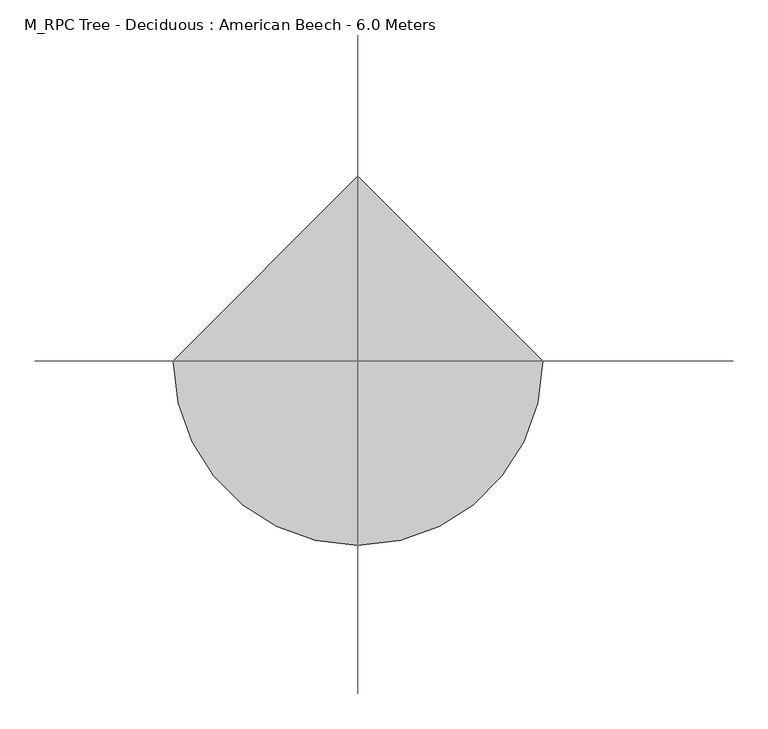
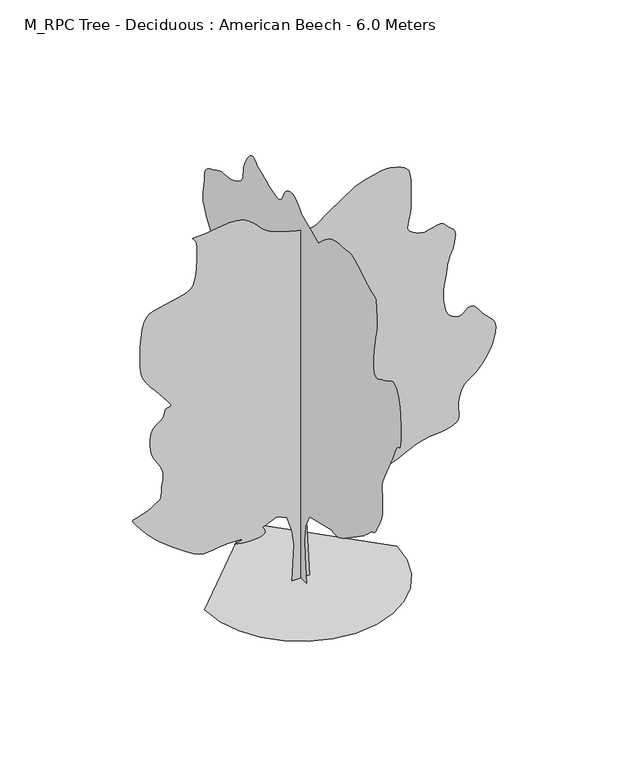
"""IFC4 building model written with IfcOpenShell, lengths in millimetres: geographic element geometry, M_RPC Tree - Deciduous : American Beech - 6.0 Meters."""

from ifc_helpers import new_model, si_unit, origin, place, context, project, spatial, triangles, source, transform, mapped, element, save


def m_rpc_tree_deciduous_american_beech_6_0_meters_be49fed4(model_context):
    return source(origin(), model_context, "Body", "Tessellation", [
        triangles([(0.0009733, 134.7013619, 0.0), (0.0009733, -147.494867, 0.0), (0.0009733, -109.8685844, 413.8878181), (0.0009733, -100.4623272, 649.050499), (0.0009733, -119.2748508, 884.2131798), (0.0009733, -232.153435, 1100.5634188), (0.0009733, -805.9506603, 1241.6609837), (0.0009733, -836.5581671, 1230.0334957), (0.0009733, -869.3831984, 1221.2035114), (0.0009733, -906.6532345, 1217.965991), (0.0009733, -950.5882708, 1223.1234524), (0.0009733, -1003.4058317, 1239.4685303), (0.0009733, -1067.3308542, 1269.7985104), (0.0009733, -1144.5859497, 1316.9135124), (0.0009733, -1455.0011593, 1533.2636787), (0.0009733, -1498.8811844, 1564.1163013), (0.0009733, -1542.2661816, 1593.486311), (0.0009733, -1585.8162849, 1623.3513485), (0.0009733, -1630.1888672, 1655.6862934), (0.0009733, -1676.041301, 1692.4613743), (0.0009733, -1724.0338657, 1735.6539413), (0.0009733, -1774.8239342, 1787.2388741), (0.0009733, -1818.8389801, 1828.7590141), (0.0009733, -1849.3615356, 1847.5739994), (0.0009733, -1871.3289448, 1854.3740204), (0.0009733, -1889.6765167, 1859.8590054), (0.0009733, -1909.3389793, 1874.7240864), (0.0009733, -1935.2541126, 1909.6614887), (0.0009733, -1972.3591152, 1975.3715767), (0.0009733, -2012.7566494, 2050.40159), (0.0009733, -2045.5841515, 2111.4491718), (0.0009733, -2071.3341785, 2166.4067184), (0.0009733, -2090.5042294, 2223.1767998), (0.0009733, -2103.5867157, 2289.651812), (0.0009733, -2111.0717239, 2373.7344704), (0.0009733, -2113.4592236, 2483.3219673), (0.0009733, -2108.7967175, 2583.5521866), (0.0009733, -2099.1991928, 2645.9521568), (0.0009733, -2091.2441551, 2687.927211), (0.0009733, -2091.5191383, 2726.9521545), (0.0009733, -2106.6016479, 2780.4523773), (0.0009733, -2143.0767471, 2865.9023941), (0.0009733, -2207.5242668, 3000.6773071), (0.0009733, -2272.3543213, 3131.8524399), (0.0009733, -2311.5169018, 3208.0527306), (0.0009733, -2333.894315, 3249.2275429), (0.0009733, -2348.3743904, 3275.2526985), (0.0009733, -2363.8419056, 3306.0525627), (0.0009733, -2389.1819286, 3361.5276649), (0.0009733, -2433.2795277, 3461.6026611), (0.0009733, -2483.0818657, 3552.8029083), (0.0009733, -2520.7019531, 3587.7528099), (0.0009733, -2547.8020432, 3595.3779259), (0.0009733, -2566.002095, 3604.6529411), (0.0009733, -2576.9770065, 3644.5278328), (0.0009733, -2582.3519691, 3743.9531593), (0.0009733, -2583.7771729, 3931.9283134), (0.0009733, -2574.1771774, 4144.4034256), (0.0009733, -2548.4520035, 4302.6033623), (0.0009733, -2511.2269501, 4413.2285866), (0.0009733, -2467.0668549, 4483.053685), (0.0009733, -2420.6095161, 4518.8035378), (0.0009733, -2376.4569786, 4527.2536034), (0.0009733, -2339.2143391, 4515.1287621), (0.0009733, -2306.9368034, 4495.0285355), (0.0009733, -2274.4943069, 4475.2535797), (0.0009733, -2241.7217434, 4456.1535828), (0.0009733, -2208.456768, 4438.0035278), (0.0009733, -2174.5318039, 4421.2036812), (0.0009733, -2139.7866863, 4406.0284447), (0.0009733, -2104.0516582, 4392.8536674), (0.0009733, -2063.4092262, 4373.6786751), (0.0009733, -2017.3366024, 4348.9034431), (0.0009733, -1970.769096, 4331.3786407), (0.0009733, -1928.6465218, 4333.9284851), (0.0009733, -1895.9015728, 4369.4036453), (0.0009733, -1877.4714478, 4450.6036308), (0.0009733, -1878.294072, 4590.37882), (0.0009733, -1893.3515831, 4743.5287743), (0.0009733, -1912.3565277, 4862.9290443), (0.0009733, -1932.3490574, 4958.6287262), (0.0009733, -1950.3665623, 5040.6789505), (0.0009733, -1963.4490486, 5119.1293945), (0.0009733, -1968.6315811, 5203.9794479), (0.0009733, -1962.9540207, 5305.2790787), (0.0009733, -1955.0840069, 5402.479541), (0.0009733, -1951.8190899, 5472.3543457), (0.0009733, -1947.4040977, 5521.0042831), (0.0009733, -1936.0790623, 5554.5045639), (0.0009733, -1912.0815445, 5578.9792328), (0.0009733, -1869.6565178, 5600.4796646), (0.0009733, -1803.044014, 5625.1043243), (0.0009733, -1720.9064404, 5661.3794357), (0.0009733, -1636.6338226, 5709.179425), (0.0009733, -1551.5337845, 5761.6047134), (0.0009733, -1466.931245, 5811.7045624), (0.0009733, -1384.1386242, 5852.5799744), (0.0009733, -1304.4711033, 5877.3546249), (0.0009733, -1229.2460438, 5879.0795197), (0.0009733, -1155.7484224, 5869.4295273), (0.0009733, -1081.2633614, 5862.9049255), (0.0009733, -1007.1082947, 5856.8547134), (0.0009733, -934.5982584, 5848.679631), (0.0009733, -865.0506866, 5835.7548386), (0.0009733, -799.7806154, 5815.4049179), (0.0009733, -740.1056242, 5785.0044479), (0.0009733, -686.9580688, 5749.2798843), (0.0009733, -639.7330444, 5714.5296799), (0.0009733, -597.445473, 5680.604425), (0.0009733, -559.105444, 5647.3547104), (0.0009733, -523.727916, 5614.5793854), (0.0009733, -490.3254127, 5582.1296219), (0.0009733, -457.9103854, 5549.8542664), (0.0009733, -15.8033629, 5737.9794113), (0.0009733, 22.480868, 5779.9547562), (0.0009733, 60.6828013, 5819.9046432), (0.0009733, 98.7203278, 5855.7047836), (0.0009733, 136.5108627, 5885.354718), (0.0009733, 173.9723933, 5906.7795731), (0.0009733, 211.0226754, 5917.9050568), (0.0009733, 247.5792013, 5916.7045486), (0.0009733, 282.6827272, 5907.9045044), (0.0009733, 315.3177446, 5896.9545914), (0.0009733, 345.3202738, 5882.8798691), (0.0009733, 372.5252993, 5864.7048157), (0.0009733, 396.7678239, 5841.4294922), (0.0009733, 417.8828505, 5812.054541), (0.0009733, 435.7103597, 5775.6044403), (0.0009733, 452.7128829, 5735.1795822), (0.0009733, 472.6778707, 5696.4046234), (0.0009733, 497.4153869, 5662.079393), (0.0009733, 528.7329157, 5634.979303), (0.0009733, 568.4429555, 5617.9047638), (0.0009733, 618.3554976, 5613.7044388), (0.0009733, 680.2805695, 5625.1043243), (0.0009733, 747.7156248, 5646.6297546), (0.0009733, 813.1781261, 5670.6294525), (0.0009733, 876.993199, 5696.6796066), (0.0009733, 939.4932358, 5724.37966), (0.0009733, 1001.0058329, 5753.3046387), (0.0009733, 1061.8608393, 5783.054567), (0.0009733, 1122.385924, 5813.2294693), (0.0009733, 1150.6609423, 5838.9296448), (0.0009733, 1179.2634842, 5861.5800064), (0.0009733, 1208.5259422, 5878.1545761), (0.0009733, 1238.7735146, 5885.5797043), (0.0009733, 1270.3410645, 5880.8299942), (0.0009733, 1303.5511013, 5860.8794678), (0.0009733, 1338.7360176, 5822.6294769), (0.0009733, 1373.2086227, 5775.8044281), (0.0009733, 1403.7311783, 5731.2548218), (0.0009733, 1429.8111271, 5687.8795624), (0.0009733, 1450.9562027, 5644.4793045), (0.0009733, 1466.6712318, 5599.9546967), (0.0009733, 1476.4611866, 5553.1046494), (0.0009733, 1479.8336552, 5502.8042313), (0.0009733, 1483.4812523, 5452.1044189), (0.0009733, 1495.191148, 5404.7044052), (0.0009733, 1516.1161789, 5360.4042023), (0.0009733, 1547.4087456, 5319.0793991), (0.0009733, 1590.2163071, 5280.554425), (0.0009733, 1645.6963509, 5244.6542908), (0.0009733, 1714.996336, 5211.204007), (0.0009733, 1788.9065048, 5186.2043701), (0.0009733, 1858.2064899, 5172.3790512), (0.0009733, 1924.0515987, 5164.8039322), (0.0009733, 1987.5940865, 5158.5543137), (0.0009733, 2049.9841736, 5148.679335), (0.0009733, 2112.3742607, 5130.2542969), (0.0009733, 2175.9167484, 5098.32892), (0.0009733, 2240.5017597, 5064.3292511), (0.0009733, 2303.2743816, 5038.2291), (0.0009733, 2361.2769459, 5012.9289001), (0.0009733, 2411.5469879, 4981.4040802), (0.0009733, 2451.1195724, 4936.5289124), (0.0009733, 2477.0345604, 4871.2538269), (0.0009733, 2486.331958, 4778.503965), (0.0009733, 2492.5844833, 4683.078685), (0.0009733, 2506.4019539, 4608.2036041), (0.0009733, 2520.4019714, 4544.5287117), (0.0009733, 2527.1521408, 4482.6537094), (0.0009733, 2519.2520416, 4413.2285866), (0.0009733, 2489.2945679, 4326.8286278), (0.0009733, 2429.8919437, 4214.1285301), (0.0009733, 2356.3968658, 4101.0031677), (0.0009733, 2289.9743214, 4014.028244), (0.0009733, 2231.9442879, 3944.8531059), (0.0009733, 2183.6218014, 3885.0282692), (0.0009733, 2146.3266941, 3826.2030807), (0.0009733, 2121.3692059, 3759.9780533), (0.0009733, 2110.0716396, 3677.9528275), (0.0009733, 2115.5842392, 3588.602758), (0.0009733, 2136.8916595, 3505.6778778), (0.0009733, 2169.0617889, 3428.6526375), (0.0009733, 2207.1542313, 3357.0776459), (0.0009733, 2246.2317879, 3290.4526428), (0.0009733, 2281.3643818, 3228.2526604), (0.0009733, 2307.6092915, 3170.0024368), (0.0009733, 2333.0293968, 3130.6025162), (0.0009733, 2364.704353, 3115.0525932), (0.0009733, 2396.2144936, 3108.0524391), (0.0009733, 2421.1445126, 3094.3024063), (0.0009733, 2433.074453, 3058.5275551), (0.0009733, 2425.586974, 2985.3773689), (0.0009733, 2392.2669147, 2859.5771988), (0.0009733, 2346.3593971, 2717.8521286), (0.0009733, 2303.741795, 2602.2772064), (0.0009733, 2261.946817, 2505.6519997), (0.0009733, 2218.506736, 2420.6845116), (0.0009733, 2170.9542606, 2340.1668972), (0.0009733, 2116.8167221, 2256.8517792), (0.0009733, 2053.6316254, 2163.5018085), (0.0009733, 1990.2540985, 2069.4091507), (0.0009733, 1937.0790012, 1987.8215435), (0.0009733, 1893.941518, 1917.4240963), (0.0009733, 1860.6740719, 1856.8965408), (0.0009733, 1837.1164982, 1804.928928), (0.0009733, 1823.1039814, 1760.1989548), (0.0009733, 1818.4689445, 1721.3939106), (0.0009733, 1822.4189941, 1694.76385), (0.0009733, 1831.633984, 1682.286414), (0.0009733, 1842.1640099, 1676.2263187), (0.0009733, 1850.0614929, 1668.8488621), (0.0009733, 1851.3789997, 1652.4213764), (0.0009733, 1842.1640099, 1619.2113396), (0.0009733, 1818.4689445, 1561.4837585), (0.0009733, 1798.7513981, 1500.5736683), (0.0009733, 1796.6388817, 1458.9161819), (0.0009733, 1800.9439968, 1430.4235897), (0.0009733, 1800.4789089, 1409.0036762), (0.0009733, 1784.0514233, 1388.5736732), (0.0009733, 1740.4738506, 1363.0410748), (0.0009733, 1658.5587925, 1326.3210777), (0.0009733, 1569.2912762, 1288.8036003), (0.0009733, 1504.2137077, 1262.3110313), (0.0009733, 1452.9586967, 1242.8959373), (0.0009733, 1405.1587074, 1226.6059433), (0.0009733, 1350.4460587, 1209.4934704), (0.0009733, 1278.4585922, 1187.608469), (0.0009733, 1178.8259382, 1157.003433), (0.0009733, 1078.8083513, 1127.6584219), (0.0009733, 1006.4358067, 1109.9959099), (0.0009733, 952.4932417, 1100.7283796), (0.0009733, 907.7632685, 1096.558358), (0.0009733, 863.0356934, 1094.2008711), (0.0009733, 809.0906576, 1090.3609165), (0.0009733, 736.7181129, 1081.7509043), (0.0009733, 652.0605623, 1068.0108273), (0.0009733, 567.4004683, 1051.3083584), (0.0009733, 482.7428813, 1032.140851), (0.0009733, 398.0828236, 1010.9958481), (0.0009733, 313.4252366, 988.3707756), (0.0009733, 228.7664324, 964.7582634), (0.0009733, 144.1076192, 940.6532667), (134.0396109, 0.0003104, 0.0138465), (-129.3426047, 0.0003104, 0.0138465), (-101.123079, 0.0002775, 554.9979549), (-129.3426047, 0.000265, 780.7556139), (-204.5949064, 0.0002508, 1015.9182947), (-355.1002728, 0.0002461, 1091.1708961), (-571.4504754, 0.0002508, 997.1057802), (-553.8429382, 0.0002524, 972.9983128), (-539.4454522, 0.000254, 949.3882713), (-531.465416, 0.0002555, 926.7632715), (-533.1104465, 0.0002571, 905.6181959), (-547.5904492, 0.0002587, 886.4482178), (-578.1129684, 0.0002587, 869.7482197), (-627.8879826, 0.0002602, 856.0082153), (-686.4380424, 0.0002602, 846.9307171), (-741.5356241, 0.0002602, 843.2831926), (-793.7506056, 0.0002602, 844.1606827), (-843.663184, 0.0002602, 848.6581553), (-891.8482515, 0.0002602, 855.8707237), (-938.8807732, 0.0002587, 864.8932108), (-985.3357864, 0.0002587, 874.8207298), (-938.2757229, 0.0002587, 886.8056814), (-899.1157585, 0.0002571, 898.1307169), (-875.7482168, 0.0002571, 908.1407164), (-876.0782112, 0.0002555, 916.1757637), (-908.000754, 0.0002555, 921.5782682), (-979.4132555, 0.0002555, 923.690712), (-1098.2134169, 0.0002555, 921.8532515), (-1223.378524, 0.0002571, 913.21577), (-1316.2934921, 0.0002571, 899.9682501), (-1388.4736794, 0.0002571, 889.0257494), (-1451.4387314, 0.0002571, 887.2982386), (-1516.7087299, 0.0002571, 901.6957609), (-1595.8012859, 0.0002555, 939.1307579), (-1700.2313942, 0.0002508, 1006.5108021), (-1816.016478, 0.0002461, 1088.4284037), (-1921.6016029, 0.0002414, 1165.4084433), (-2017.1466431, 0.0002367, 1238.2735451), (-2102.8191753, 0.0002336, 1307.8509842), (-2178.7867767, 0.0002289, 1374.9560452), (-2245.2068504, 0.0002242, 1440.4186192), (-2302.2492989, 0.0002211, 1505.0587143), (-2354.1368294, 0.0002179, 1567.5838223), (-2402.8969345, 0.0002132, 1625.1763824), (-2445.4045143, 0.0002101, 1676.3488403), (-2478.5321434, 0.0002085, 1719.6239605), (-2499.1544312, 0.0002069, 1753.5214554), (-2504.1520912, 0.0002054, 1776.5590027), (-2490.3793854, 0.0002038, 1787.2539894), (-2459.3920326, 0.0002038, 1794.0263958), (-2417.5419708, 0.0002038, 1805.7364368), (-2368.9443558, 0.0002022, 1821.5614883), (-2317.716814, 0.0002007, 1840.6764553), (-2267.9692692, 0.0001991, 1862.2590042), (-2223.8167316, 0.0001991, 1885.4865108), (-2189.3717411, 0.0001975, 1909.5391125), (-2162.3867603, 0.000196, 1927.8015152), (-2138.1966671, 0.000196, 1938.169051), (-2117.2992508, 0.0001944, 1946.561562), (-2100.1866325, 0.0001944, 1958.9016518), (-2087.3541309, 0.0001928, 1981.1165749), (-2079.291687, 0.0001897, 2019.1266094), (-2076.4941833, 0.0001866, 2078.8566845), (-2072.5992176, 0.0001834, 2146.7042873), (-2063.7692333, 0.0001787, 2206.9817127), (-2054.2791149, 0.0001756, 2262.4893711), (-2048.4115952, 0.0001725, 2316.0218594), (-2050.4417038, 0.0001693, 2370.3769718), (-2064.6466507, 0.0001662, 2428.3494507), (-2095.3066978, 0.0001615, 2492.7420319), (-2134.2492336, 0.0001583, 2555.8271347), (-2169.5717869, 0.0001552, 2611.5022247), (-2199.9567055, 0.0001521, 2665.0271553), (-2224.0918602, 0.0001489, 2721.6771858), (-2240.6543667, 0.0001442, 2786.727285), (-2248.3342758, 0.0001395, 2865.4274231), (-2245.8117554, 0.0001348, 2963.0772766), (-2228.8892418, 0.0001286, 3053.9275452), (-2197.981826, 0.0001254, 3115.1525871), (-2158.6842247, 0.0001223, 3156.3276901), (-2116.5866489, 0.0001207, 3186.952565), (-2077.289193, 0.0001191, 3216.6024994), (-2046.3816319, 0.000116, 3254.8024933), (-2029.4615891, 0.0001129, 3311.1025452), (-2011.7716805, 0.0001113, 3359.2778023), (-1982.4016708, 0.0001097, 3377.3028648), (-1952.6991234, 0.0001097, 3381.2026268), (-1934.0241005, 0.0001082, 3386.9028603), (-1937.7266361, 0.0001082, 3410.3778809), (-1975.1615604, 0.0001035, 3467.6028763), (-2057.6791981, 9.72e-05, 3574.5027466), (-2156.9017754, 9.09e-05, 3694.6029739), (-2237.5292667, 8.47e-05, 3789.0530228), (-2300.5494026, 8e-05, 3870.1780128), (-2346.9519482, 7.53e-05, 3950.303064), (-2377.7218723, 7.05e-05, 4041.8032928), (-2393.8469055, 6.27e-05, 4156.9782394), (-2396.3144875, 5.33e-05, 4308.2036018), (-2391.2694466, 4.39e-05, 4470.0786049), (-2382.4394623, 3.61e-05, 4609.2538307), (-2367.1893757, 2.98e-05, 4726.0536781), (-2342.8918762, 2.35e-05, 4820.8039993), (-2306.911805, 1.88e-05, 4893.8541916), (-2256.6142937, 1.57e-05, 4945.4789474), (-2189.3717411, 1.41e-05, 4976.0538254), (-2104.7392616, 1.25e-05, 4994.8788391), (-2008.7541321, 1.25e-05, 5012.5289246), (-1908.491502, 1.1e-05, 5031.3539383), (-1811.0265209, 9.4e-06, 5053.6293228), (-1723.4339024, 7.8e-06, 5081.6543564), (-1652.7887959, 6.3e-06, 5117.7288986), (-1606.1663509, 3.1e-06, 5164.2039688), (-1578.8513031, -1.6e-06, 5232.7044388), (-1560.4237942, -6.3e-06, 5326.3795349), (-1549.3987404, -1.25e-05, 5434.7043182), (-1544.298761, -2.04e-05, 5547.1544312), (-1543.6387722, -2.67e-05, 5653.1793549), (-1545.9437187, -3.14e-05, 5742.2547318), (-1549.7288074, -3.45e-05, 5803.8294617), (-1560.9438206, -3.76e-05, 5842.6799973), (-1580.7187763, -3.92e-05, 5871.4799835), (-1600.3263004, -4.08e-05, 5891.7049118), (-1611.0487564, -4.08e-05, 5904.879689), (-1604.1663277, -4.23e-05, 5912.4298096), (-1570.95382, -4.23e-05, 5915.9045975), (-1502.6962132, -4.23e-05, 5916.7295471), (-1406.2711395, -4.23e-05, 5923.0547424), (-1298.001004, -4.39e-05, 5937.4550262), (-1183.3109842, -4.39e-05, 5953.0046585), (-1067.6358501, -4.39e-05, 5962.7796432), (-956.4032501, -4.39e-05, 5959.9048187), (-855.043158, -4.39e-05, 5937.4550262), (-768.9856201, -4.08e-05, 5888.5045258), (-703.6355392, -3.61e-05, 5829.3546478), (-655.0655388, -3.29e-05, 5779.2298004), (-614.7254866, -3.14e-05, 5735.7045502), (-574.0554763, -2.82e-05, 5696.3046295), (-524.5004342, -2.67e-05, 5658.5546082), (-457.5028522, -2.35e-05, 5619.9546387), (-364.5052946, -2.19e-05, 5578.0792877), (-256.7552037, -1.88e-05, 5538.7543625), (-153.2841212, -1.72e-05, 5508.8044464), (-57.2167973, -1.57e-05, 5487.254599), (28.3195219, -1.57e-05, 5473.1042999), (100.1988349, -1.57e-05, 5465.3791901), (155.2941184, -1.41e-05, 5463.054332), (190.4793981, -1.57e-05, 5465.2042007), (215.8194211, -1.57e-05, 5473.054303), (243.4629554, -1.57e-05, 5487.6295761), (273.410219, -1.72e-05, 5507.6545166), (305.6602309, -1.88e-05, 5531.7792068), (340.2152802, -2.04e-05, 5558.729306), (377.0728051, -2.19e-05, 5587.1293167), (416.2353493, -2.35e-05, 5615.7043167), (792.4981384, -3.92e-05, 5869.679512), (817.288195, -3.92e-05, 5878.9295288), (882.5581936, -4.08e-05, 5902.1548553), (974.6482847, -4.23e-05, 5932.6297394), (1079.9033426, -4.55e-05, 5963.5795944), (1184.6634453, -4.55e-05, 5988.3048294), (1275.2734669, -4.7e-05, 6000.0046967), (1338.0760288, -4.7e-05, 5991.9796051), (1385.3260517, -4.55e-05, 5975.0550568), (1436.1986732, -4.39e-05, 5961.4297256), (1487.4012165, -4.39e-05, 5946.3050674), (1535.6386791, -4.23e-05, 5924.9546265), (1577.6262325, -4.08e-05, 5892.5548599), (1610.068729, -3.76e-05, 5844.3798935), (1629.6788692, -3.29e-05, 5775.6294388), (1639.0838184, -2.82e-05, 5698.6044891), (1643.8838161, -2.51e-05, 5627.2047775), (1645.2263214, -2.04e-05, 5558.9042953), (1644.2663509, -1.72e-05, 5491.2793533), (1642.1538345, -1.25e-05, 5421.8545212), (1640.0437889, -7.8e-06, 5348.1293701), (1639.0838184, -3.1e-06, 5267.6790482), (1634.0913906, 1.6e-06, 5187.5792862), (1622.1912449, 6.3e-06, 5116.5539703), (1607.9838272, 9.4e-06, 5054.4042755), (1596.081356, 1.25e-05, 5001.0040466), (1591.0912537, 1.57e-05, 4956.1288788), (1597.6187622, 1.72e-05, 4919.6537796), (1620.2713039, 1.88e-05, 4891.4037598), (1651.9738747, 2.04e-05, 4868.9289688), (1682.6888603, 2.19e-05, 4849.728978), (1712.5813671, 2.19e-05, 4833.6537964), (1741.8138851, 2.35e-05, 4820.5540146), (1770.5564621, 2.35e-05, 4810.2287727), (1798.9665012, 2.51e-05, 4802.5539505), (1827.213905, 2.51e-05, 4797.3289787), (1863.2490601, 2.51e-05, 4800.3037971), (1911.6264851, 2.35e-05, 4812.9788956), (1967.4066559, 2.35e-05, 4828.9287941), (2025.6565887, 2.19e-05, 4841.7788818), (2081.4366142, 2.19e-05, 4845.0539726), (2129.8141846, 2.35e-05, 4832.3788742), (2165.8491943, 2.51e-05, 4797.3289787), (2195.3593117, 2.67e-05, 4758.0787582), (2225.6892918, 2.82e-05, 4731.9538994), (2254.2093533, 2.98e-05, 4711.4536972), (2278.2892788, 3.14e-05, 4688.9539078), (2295.2918747, 3.29e-05, 4656.9288277), (2302.5869236, 3.61e-05, 4607.7786301), (2297.5418827, 4.08e-05, 4533.9537758), (2283.3617889, 4.55e-05, 4455.6536133), (2265.8943958, 4.86e-05, 4393.6536186), (2246.4493618, 5.17e-05, 4341.2036224), (2226.3468098, 5.49e-05, 4291.5284569), (2206.9042465, 5.8e-05, 4237.9035324), (2189.4342373, 6.27e-05, 4173.6033875), (2175.2567596, 6.74e-05, 4091.8534355), (2162.3117649, 7.21e-05, 4004.3782516), (2148.874213, 7.68e-05, 3925.278138), (2136.7516972, 8.15e-05, 3851.452993), (2127.756752, 8.62e-05, 3779.753009), (2123.6991508, 8.94e-05, 3707.0780846), (2126.3867775, 9.41e-05, 3630.302829), (2137.6292599, 9.88e-05, 3546.2777252), (2155.4842747, 0.0001035, 3469.5027603), (2176.791695, 0.0001066, 3413.652681), (2201.5542824, 0.0001097, 3374.2527603), (2229.7743622, 0.0001113, 3346.8526886), (2261.4493183, 0.0001129, 3327.0277359), (2296.5819122, 0.0001129, 3310.302594), (2335.1669117, 0.0001144, 3292.3025299), (2374.57439, 0.0001144, 3289.8526794), (2413.1620056, 0.0001129, 3313.0777153), (2452.4043777, 0.0001113, 3347.3276596), (2493.7896423, 0.0001097, 3377.9778236), (2538.8020111, 0.0001082, 3390.3276512), (2588.9021507, 0.0001097, 3369.8027412), (2645.5771797, 0.0001144, 3301.7025375), (2706.5522369, 0.0001191, 3218.4776756), (2765.8771042, 0.0001223, 3156.4526825), (2819.5773148, 0.0001254, 3106.9525063), (2863.7772331, 0.0001286, 3061.2523888), (2894.4523956, 0.0001317, 3010.6025734), (2907.702459, 0.0001348, 2946.27743), (2899.552375, 0.0001411, 2859.6021973), (2878.1022308, 0.0001458, 2766.3523659), (2853.5522758, 0.0001505, 2686.1020317), (2825.0272728, 0.0001552, 2615.752256), (2791.7272705, 0.0001583, 2552.1270699), (2752.8273193, 0.0001615, 2492.1121284), (2707.5271774, 0.0001662, 2432.6019527), (2654.9771873, 0.0001693, 2370.4569088), (2600.8270042, 0.0001725, 2317.1443199), (2551.1021324, 0.0001756, 2280.2868313), (2505.6519997, 0.0001772, 2250.9967587), (2464.3344635, 0.0001787, 2220.3917953), (2426.9544777, 0.0001803, 2179.5842571), (2393.3594353, 0.000185, 2119.691692), (2363.3868462, 0.0001897, 2031.8240902), (2347.2343437, 0.000196, 1934.7965824), (2348.1944595, 0.0002007, 1852.2490047), (2355.7344063, 0.0002038, 1782.5363995), (2359.3269196, 0.0002085, 1724.0139542), (2348.4393574, 0.0002116, 1675.0338043), (2312.5418392, 0.0002132, 1633.9512829), (2241.1018684, 0.0002148, 1599.1237576), (2155.26423, 0.0002164, 1575.9487186), (2078.4766205, 0.0002179, 1565.7737583), (2003.661565, 0.0002179, 1560.866209), (1923.7465302, 0.0002179, 1553.4887524), (1831.6565117, 0.0002195, 1535.9111916), (1720.3138893, 0.0002211, 1500.3962082), (1582.6438042, 0.0002258, 1439.2111347), (1432.7436516, 0.0002289, 1368.8411568), (1291.0710491, 0.000232, 1310.483527), (1160.0909626, 0.0002352, 1263.4785473), (1042.2783136, 0.0002383, 1227.1685543), (940.0957426, 0.0002399, 1200.8959574), (856.0131569, 0.0002399, 1184.0009857), (792.4981384, 0.0002414, 1175.8284468), (397.4228348, 0.0002414, 1166.4234249), (105.8200852, 0.0002446, 1119.3909033), (87.0075707, 0.0002587, 865.4131645), (-1430.8636791, 0.0, 0.0118397), (-1393.0361916, -327.8602567, 0.0118397), (-1285.305994, -628.9454762, 0.0118397), (-1116.2958887, -894.633256, 0.0118397), (-894.633256, -1116.2958887, 0.0118397), (-628.9454762, -1285.305994, 0.0118397), (-327.8602567, -1393.0361916, 0.0118397), (6.25e-05, -1430.8636791, 0.0118397), (327.8602567, -1393.0361916, 0.0118397), (628.9454762, -1285.305994, 0.0118397), (894.633256, -1116.2958887, 0.0118397), (1116.2958887, -894.633256, 0.0118397), (1285.305994, -628.9454762, 0.0118397), (1393.0361916, -327.8602567, 0.0118397), (1430.8636791, 0.0001254, 0.0118397), (-0.0001876, 1430.8636791, 0.0118397)], [[1, 2, 3], [254, 1, 3], [254, 3, 4], [254, 4, 5], [254, 5, 6], [53, 54, 55], [52, 53, 55], [201, 202, 203], [201, 203, 204], [200, 201, 204], [222, 223, 224], [52, 55, 56], [200, 204, 205], [199, 200, 205], [253, 254, 6], [221, 222, 224], [221, 224, 225], [229, 230, 231], [229, 231, 232], [228, 229, 232], [228, 232, 233], [227, 228, 233], [252, 253, 6], [221, 225, 226], [220, 221, 226], [199, 205, 206], [198, 199, 206], [62, 63, 64], [61, 62, 64], [61, 64, 65], [60, 61, 65], [60, 65, 66], [59, 60, 66], [59, 66, 67], [59, 67, 68], [58, 59, 68], [58, 68, 69], [58, 69, 70], [57, 58, 70], [57, 70, 71], [57, 71, 72], [57, 72, 73], [57, 73, 74], [56, 57, 74], [52, 56, 74], [51, 52, 74], [50, 51, 74], [50, 74, 75], [49, 50, 75], [48, 49, 75], [47, 48, 75], [46, 47, 75], [45, 46, 75], [44, 45, 75], [43, 44, 75], [42, 43, 75], [42, 75, 76], [41, 42, 76], [227, 233, 234], [226, 227, 234], [220, 226, 234], [219, 220, 234], [219, 234, 235], [219, 235, 236], [219, 236, 237], [218, 219, 237], [218, 237, 238], [218, 238, 239], [218, 239, 240], [217, 218, 240], [217, 240, 241], [217, 241, 242], [217, 242, 243], [217, 243, 244], [217, 244, 245], [217, 245, 246], [216, 217, 246], [216, 246, 247], [215, 216, 247], [215, 247, 248], [251, 252, 6], [88, 89, 90], [88, 90, 91], [87, 88, 91], [87, 91, 92], [86, 87, 92], [86, 92, 93], [85, 86, 93], [84, 85, 93], [84, 93, 94], [83, 84, 94], [82, 83, 94], [81, 82, 94], [81, 94, 95], [80, 81, 95], [80, 95, 96], [80, 96, 97], [80, 97, 98], [80, 98, 99], [80, 99, 100], [80, 100, 101], [80, 101, 102], [80, 102, 103], [80, 103, 104], [80, 104, 105], [80, 105, 106], [80, 106, 107], [80, 107, 108], [80, 108, 109], [80, 109, 110], [80, 110, 111], [80, 111, 112], [79, 80, 112], [79, 112, 113], [78, 79, 113], [77, 78, 113], [76, 77, 113], [41, 76, 113], [40, 41, 113], [40, 113, 114], [39, 40, 114], [198, 206, 207], [197, 198, 207], [196, 197, 207], [196, 207, 208], [195, 196, 208], [195, 208, 209], [195, 209, 210], [195, 210, 211], [194, 195, 211], [194, 211, 212], [194, 212, 213], [193, 194, 213], [193, 213, 214], [214, 215, 248], [193, 214, 248], [193, 248, 249], [192, 193, 249], [192, 249, 250], [192, 250, 251], [192, 251, 6], [192, 6, 7], [191, 192, 7], [190, 191, 7], [189, 190, 7], [38, 39, 114], [37, 38, 114], [36, 37, 114], [35, 36, 114], [34, 35, 114], [33, 34, 114], [32, 33, 114], [31, 32, 114], [30, 31, 114], [29, 30, 114], [28, 29, 114], [27, 28, 114], [26, 27, 114], [25, 26, 114], [24, 25, 114], [23, 24, 114], [22, 23, 114], [21, 22, 114], [20, 21, 114], [19, 20, 114], [18, 19, 114], [17, 18, 114], [16, 17, 114], [15, 16, 114], [14, 15, 114], [13, 14, 114], [12, 13, 114], [11, 12, 114], [10, 11, 114], [9, 10, 114], [8, 9, 114], [7, 8, 114], [189, 7, 114], [188, 189, 114], [188, 114, 115], [188, 115, 116], [188, 116, 117], [188, 117, 118], [188, 118, 119], [188, 119, 120], [188, 120, 121], [146, 147, 148], [145, 146, 148], [144, 145, 148], [144, 148, 149], [143, 144, 149], [143, 149, 150], [142, 143, 150], [142, 150, 151], [142, 151, 152], [141, 142, 152], [141, 152, 153], [141, 153, 154], [141, 154, 155], [141, 155, 156], [140, 141, 156], [140, 156, 157], [139, 140, 157], [138, 139, 157], [138, 157, 158], [137, 138, 158], [137, 158, 159], [136, 137, 159], [135, 136, 159], [135, 159, 160], [134, 135, 160], [134, 160, 161], [174, 175, 176], [173, 174, 176], [173, 176, 177], [172, 173, 177], [171, 172, 177], [171, 177, 178], [170, 171, 178], [170, 178, 179], [169, 170, 179], [168, 169, 179], [167, 168, 179], [166, 167, 179], [165, 166, 179], [165, 179, 180], [165, 180, 181], [165, 181, 182], [165, 182, 183], [165, 183, 184], [165, 184, 185], [165, 185, 186], [165, 186, 187], [164, 165, 187], [164, 187, 188], [163, 164, 188], [162, 163, 188], [161, 162, 188], [134, 161, 188], [133, 134, 188], [132, 133, 188], [125, 126, 127], [124, 125, 127], [124, 127, 128], [123, 124, 128], [122, 123, 128], [121, 122, 128], [121, 128, 129], [121, 129, 130], [121, 130, 131], [188, 121, 131], [132, 188, 131], [274, 275, 276], [531, 255, 256], [531, 256, 257], [531, 257, 258], [531, 258, 259], [530, 531, 259], [376, 377, 378], [376, 378, 379], [375, 376, 379], [273, 274, 276], [273, 276, 277], [375, 379, 380], [374, 375, 380], [273, 277, 278], [272, 273, 278], [301, 302, 303], [301, 303, 304], [300, 301, 304], [300, 304, 305], [299, 300, 305], [299, 305, 306], [298, 299, 306], [298, 306, 307], [297, 298, 307], [297, 307, 308], [271, 272, 278], [296, 297, 308], [296, 308, 309], [373, 374, 380], [373, 380, 381], [372, 373, 381], [295, 296, 309], [295, 309, 310], [294, 295, 310], [294, 310, 311], [294, 311, 312], [294, 312, 313], [293, 294, 313], [293, 313, 314], [292, 293, 314], [271, 278, 279], [291, 292, 314], [530, 259, 260], [372, 381, 382], [371, 372, 382], [291, 314, 315], [290, 291, 315], [371, 382, 383], [370, 371, 383], [370, 383, 384], [369, 370, 384], [369, 384, 385], [369, 385, 386], [369, 386, 387], [369, 387, 388], [369, 388, 389], [369, 389, 390], [368, 369, 390], [368, 390, 391], [367, 368, 391], [367, 391, 392], [367, 392, 393], [366, 367, 393], [366, 393, 394], [270, 271, 279], [366, 394, 395], [338, 339, 340], [338, 340, 341], [289, 290, 315], [483, 484, 485], [483, 485, 486], [482, 483, 486], [481, 482, 486], [481, 486, 487], [480, 481, 487], [288, 289, 315], [287, 288, 315], [286, 287, 315], [285, 286, 315], [284, 285, 315], [283, 284, 315], [282, 283, 315], [282, 315, 316], [281, 282, 316], [281, 316, 317], [281, 317, 318], [281, 318, 319], [281, 319, 320], [280, 281, 320], [280, 320, 321], [279, 280, 321], [279, 321, 322], [480, 487, 488], [264, 265, 266], [263, 264, 266], [263, 266, 267], [262, 263, 267], [262, 267, 268], [261, 262, 268], [261, 268, 269], [261, 269, 270], [261, 270, 279], [261, 279, 322], [260, 261, 322], [530, 260, 322], [530, 322, 323], [529, 530, 323], [529, 323, 324], [366, 395, 396], [365, 366, 396], [337, 338, 341], [337, 341, 342], [529, 324, 325], [528, 529, 325], [527, 528, 325], [526, 527, 325], [525, 526, 325], [524, 525, 325], [523, 524, 325], [522, 523, 325], [521, 522, 325], [521, 325, 326], [521, 326, 327], [521, 327, 328], [521, 328, 329], [521, 329, 330], [521, 330, 331], [521, 331, 332], [521, 332, 333], [521, 333, 334], [521, 334, 335], [521, 335, 336], [521, 336, 337], [521, 337, 342], [520, 521, 342], [520, 342, 343], [519, 520, 343], [518, 519, 343], [518, 343, 344], [517, 518, 344], [449, 450, 451], [448, 449, 451], [448, 451, 452], [447, 448, 452], [446, 447, 452], [446, 452, 453], [516, 517, 344], [515, 516, 344], [514, 515, 344], [513, 514, 344], [512, 513, 344], [511, 512, 344], [510, 511, 344], [509, 510, 344], [508, 509, 344], [507, 508, 344], [506, 507, 344], [505, 506, 344], [504, 505, 344], [503, 504, 344], [502, 503, 344], [501, 502, 344], [500, 501, 344], [499, 500, 344], [498, 499, 344], [497, 498, 344], [496, 497, 344], [495, 496, 344], [494, 495, 344], [493, 494, 344], [492, 493, 344], [491, 492, 344], [490, 491, 344], [489, 490, 344], [488, 489, 344], [480, 488, 344], [479, 480, 344], [478, 479, 344], [477, 478, 344], [476, 477, 344], [475, 476, 344], [474, 475, 344], [473, 474, 344], [472, 473, 344], [471, 472, 344], [470, 471, 344], [469, 470, 344], [468, 469, 344], [467, 468, 344], [466, 467, 344], [465, 466, 344], [464, 465, 344], [463, 464, 344], [463, 344, 345], [462, 463, 345], [462, 345, 346], [461, 462, 346], [460, 461, 346], [459, 460, 346], [458, 459, 346], [457, 458, 346], [456, 457, 346], [455, 456, 346], [454, 455, 346], [453, 454, 346], [446, 453, 346], [445, 446, 346], [444, 445, 346], [443, 444, 346], [442, 443, 346], [441, 442, 346], [440, 441, 346], [439, 440, 346], [438, 439, 346], [437, 438, 346], [436, 437, 346], [435, 436, 346], [435, 346, 347], [435, 347, 348], [435, 348, 349], [435, 349, 350], [435, 350, 351], [435, 351, 352], [435, 352, 353], [435, 353, 354], [435, 354, 355], [435, 355, 356], [435, 356, 357], [435, 357, 358], [435, 358, 359], [435, 359, 360], [435, 360, 361], [435, 361, 362], [435, 362, 363], [435, 363, 364], [435, 364, 365], [435, 365, 396], [435, 396, 397], [435, 397, 398], [435, 398, 399], [435, 399, 400], [435, 400, 401], [435, 401, 402], [435, 402, 403], [435, 403, 404], [435, 404, 405], [435, 405, 406], [435, 406, 407], [435, 407, 408], [435, 408, 409], [434, 435, 409], [433, 434, 409], [432, 433, 409], [431, 432, 409], [430, 431, 409], [429, 430, 409], [429, 409, 410], [429, 410, 411], [429, 411, 412], [428, 429, 412], [428, 412, 413], [427, 428, 413], [426, 427, 413], [426, 413, 414], [425, 426, 414], [425, 414, 415], [425, 415, 416], [425, 416, 417], [424, 425, 417], [424, 417, 418], [423, 424, 418], [423, 418, 419], [422, 423, 419], [422, 419, 420], [421, 422, 420], [546, 547, 532], [545, 546, 532], [545, 532, 533], [544, 545, 533], [544, 533, 534], [544, 534, 535], [543, 544, 535], [542, 543, 535], [542, 535, 536], [542, 536, 537], [542, 537, 538], [542, 538, 539], [542, 539, 540], [542, 540, 541]], closed=False),
    ])


if __name__ == "__main__":
    model = new_model("IFC4")
    model_context = context("Model", 3, world=origin())
    ifc_project = project(units=[si_unit("LENGTHUNIT", "METRE", prefix="MILLI")], contexts=[model_context])
    site = spatial("IfcSite", under=ifc_project)
    building = spatial("IfcBuilding", under=site)
    placement = place(None, origin())
    m_rpc_tree_deciduous_american_beech_6_0_meters_shape = m_rpc_tree_deciduous_american_beech_6_0_meters_be49fed4(model_context)
    element("IfcGeographicElement", 1, ObjectType="M_RPC Tree - Deciduous : American Beech - 6.0 Meters", at=placement, inside=building, context=model_context, shape_type="MappedRepresentation", body=[
        mapped(m_rpc_tree_deciduous_american_beech_6_0_meters_shape, transform((0.0, 0.0, 0.0), x_axis=(1.0, 0.0, 0.0), y_axis=(0.0, 1.0, 0.0), z_axis=(0.0, 0.0, 1.0))),
    ])
    save(model, "model.ifc")

# Revit data of these elements
# Type "M_RPC Tree - Deciduous : American Beech - 6.0 Meters"
#   built-in parameter 1005198 = "{2, 15},{39, RPC-16-G1GQ-43Q0-7NP3-0000-ST1L-LVER-AU},{1, 0},{1, 0},{2, 13},{1, 8},{5, Color},{1, 0},{1, 0},{3, 0.8},{3, 0.8},{3, 0.8},{1, 8},{7, BBoxMin},{1, 0},{1, 0},{1, 0},{1, 0},{1, 0},{1, 8},{7, BBoxMax},{1, 0},{1, 0},{1, 0},{1, 0},{1, 0},{2, 11},{9, RPCTypeId},{1, 0},{1, 0},{39, RPC-16-G1GQ-43Q0-7NP3-0000-ST1L-LVER-AU},{1, 6},{14, RPCPlantHeight},{1, 0},{1, 0},{6, 19.685},{2, 11},{7, keyword},{1, 0},{1, 0},{34, :RPCs:Trees [General]:Geometry:RPC},{2, 11},{8, category},{1, 0},{1, 0},{15, Trees [General]},{2, 11},{12, LocalizedUID},{1, 0},{1, 0},{14, American Beech},{2, 14},{6, Height},{1, 0},{1, 0},{6, 19.685},{1, 2},{16, Cast Reflections},{1, 0},{1, 0},{1, 0},{1, 2},{12, Cast Shadows},{1, 0},{1, 0},{1, 1},{1, 2},{9, Lock View},{1, 0},{1, 0},{1, 0},{1, 4},{5, ViewC},{1, 0},{1, 0},{1, 0},{21, assetlibrary_base.fbx},{1, 5},"
#   built-in parameter 1005195 = "RPC-16-G1GQ-43Q0-7NP3-0000-ST1L-LVER-AU"
#   Type Comments = "American Beech"
#   Height = 6 m
#   Default Elevation = 0
